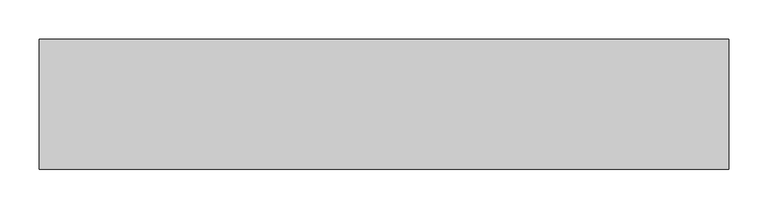
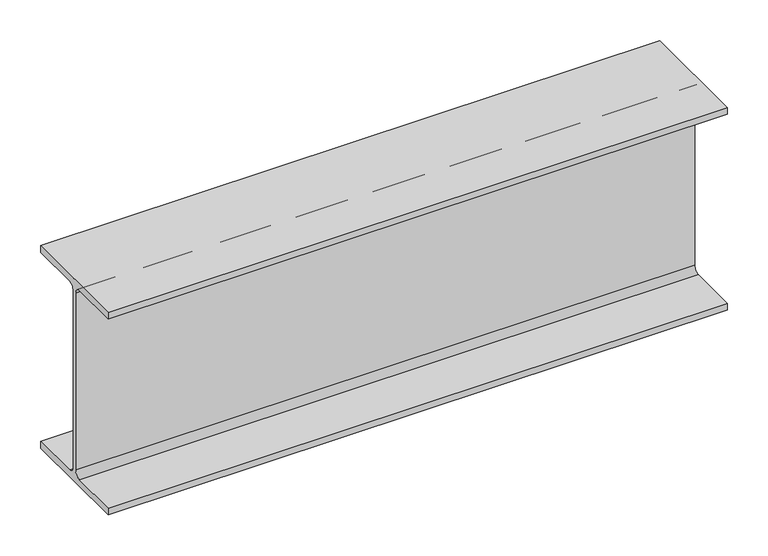
"""IFC4 building model written with IfcOpenShell, lengths in millimetres: beam geometry, Old_Steel Beam_H-KSD3502 : H_SB_ASB_H-482×300x11x15."""

from ifc_helpers import new_model, si_unit, point, frame, frame_2d, origin, place, context, project, spatial, polyline, circle_curve, trimmed, segment, composite_curve, outline, extrude, source, transform, mapped, element, save


def beam_ab6c920a(model_context):
    return source(origin(), model_context, "Body", "SweptSolid", [
        extrude(outline(composite_curve([segment(polyline([(82.5, -141.5), (82.5, -151.7), (-82.5, -151.7), (-82.5, -141.5), (-11.9, -141.5)]), True, "CONTINUOUS"), segment(trimmed(circle_curve(frame_2d((-11.9, -132.6)), 8.9), [point((-11.9, -141.5))], [point((-3.0, -132.6))], True, "CARTESIAN"), True, "CONTINUOUS"), segment(polyline([(-3.0, -132.6), (-3.0, 132.6)]), True, "CONTINUOUS"), segment(trimmed(circle_curve(frame_2d((-11.9, 132.6)), 8.9), [point((-3.0, 132.6))], [point((-11.9, 141.5))], True, "CARTESIAN"), True, "CONTINUOUS"), segment(polyline([(-11.9, 141.5), (-82.5, 141.5), (-82.5, 151.7), (82.5, 151.7), (82.5, 141.5), (11.9, 141.5)]), True, "CONTINUOUS"), segment(trimmed(circle_curve(frame_2d((11.9, 132.6)), 8.9), [point((11.9, 141.5))], [point((3.0, 132.6))], True, "CARTESIAN"), True, "CONTINUOUS"), segment(polyline([(3.0, 132.6), (3.0, -132.6)]), True, "CONTINUOUS"), segment(trimmed(circle_curve(frame_2d((11.9, -132.6)), 8.9), [point((3.0, -132.6))], [point((11.9, -141.5))], True, "CARTESIAN"), True, "CONTINUOUS"), segment(polyline([(11.9, -141.5), (82.5, -141.5)]), True, "CONTINUOUS")], self_intersect=False)), frame((-444.5, 0.0, 0.0), z_axis=(1.0, 0.0, 0.0), x_axis=(0.0, 1.0, 0.0)), (0.0, 0.0, 1.0), 876.3),
    ])


if __name__ == "__main__":
    model = new_model("IFC4")
    model_context = context("Model", 3, world=origin())
    ifc_project = project(units=[si_unit("LENGTHUNIT", "METRE", prefix="MILLI")], contexts=[model_context])
    site = spatial("IfcSite", under=ifc_project)
    building = spatial("IfcBuilding", under=site)
    placement = place(None, origin())
    beam_shape = beam_ab6c920a(model_context)
    element("IfcBeam", 1, ObjectType="Old_Steel Beam_H-KSD3502 : H_SB_ASB_H-482×300x11x15", at=placement, inside=building, context=model_context, shape_type="MappedRepresentation", body=[
        mapped(beam_shape, transform((0.0, 0.0, 0.0), x_axis=(1.0, 0.0, 0.0), y_axis=(0.0, 1.0, 0.0), z_axis=(0.0, 0.0, 1.0))),
    ])
    save(model, "model.ifc")

# Revit data of these elements
# Type "Old_Steel Beam_H-KSD3502 : H_SB_ASB_H-482×300x11x15"
#   Width = 30.0 cm
#   Web Thickness = 1.1 cm
#   Web Fillet = 2.6 cm
#   Warping Constant = 3680250.0 cm⁶
#   Torsional Moment of Inertia = 88.2192 cm⁴
#   Torsional Modulus = 1.0 cm³
#   Section Area = 145.5 cm²
#   Plastic Modulus weak axis = 695.0 cm³
#   Plastic Modulus strong axis = 2790.0 cm³
#   Perimeter = 2.10 m²/m
#   Nominal Weight = 114.00 kgf/m
#   Moment of Inertia weak axis = 6760.00 cm⁴
#   Moment of Inertia strong axis = 60400.00 cm⁴
#   Height = 48.2 cm
#   Flange Thickness = 1.5 cm
#   Elastic Modulus weak axis = 451.0 cm³
#   Elastic Modulus strong axis = 2500.0 cm³
#   Centroid Vertical = 24.1 cm
#   Centroid Horizontal = 15.0 cm
#   Length [instance default] = 1.5240 m
#   Structural Material [instance default] = Steel, 45-345
#   Assembly Code = ""
# Element 1 (IfcBeam, "Old_Steel Beam_H-KSD3502 : H_SB_ASB_H-482×300x11x15")
#   Structural Material = none
# Materials
#   "Steel, 45-345": class "Metal", colour RGB 189 187 185, transparency 0, Description = "Steel 345 MPa", Cost = 0
